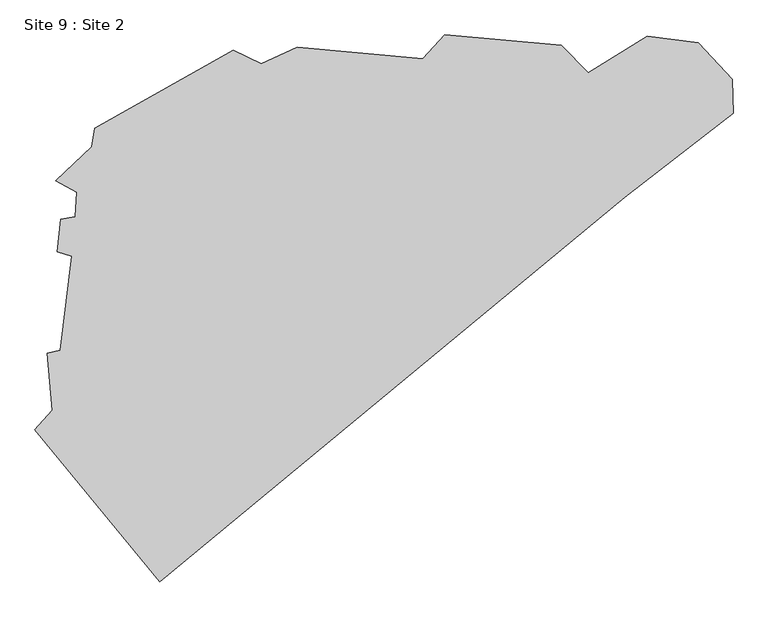
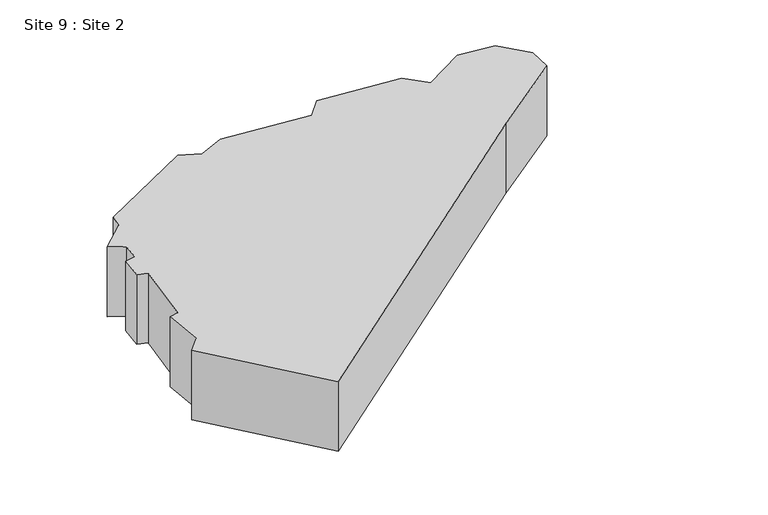
"""IFC4 building model written with IfcOpenShell, lengths in millimetres: geographic element geometry, Site 9 : Site 2."""

from ifc_helpers import new_model, si_unit, frame, origin, place, context, project, spatial, polyline, outline, extrude, source, transform, mapped, element, save


def site_9_site_2_4225363e(model_context):
    return source(origin(), model_context, "Body", "SweptSolid", [
        extrude(outline(polyline([(-52663.5762578, -39928.595116), (-61550.4941803, -29130.9188955), (-60310.8192275, -27726.3601163), (-60658.3068747, -23656.9457677), (-59741.0581441, -23467.0172822), (-58932.8015846, -16772.5268672), (-59944.2788523, -16453.0480066), (-59707.250861, -14119.4876127), (-58688.4150048, -13931.0308449), (-58561.8044455, -12205.5214874), (-60073.8708382, -11370.7058979), (-57498.8164451, -8969.4086212), (-57276.5056308, -7651.7194841), (-47441.5131213, -2104.0860833), (-45422.9695062, -3047.805243), (-42865.5757254, -1865.5534745), (-33936.0159808, -2706.1773326), (-32387.1560323, -1001.2724521), (-24065.6600225, -1731.4786944), (-22163.4249429, -3689.5973319), (-17959.9992411, -1108.6737776), (-14308.6691642, -1568.0052826), (-11907.3202968, -4143.0053853), (-11841.0507764, -6582.6105086), (-19548.5539567, -12567.4991584), (-52663.5762578, -39928.595116)])), frame((0.0, 0.0, 266395.2), z_axis=(0.0, 0.0, 1.0), x_axis=(1.0, 0.0, 0.0)), (0.0, 0.0, 1.0), 7620.0),
    ])


if __name__ == "__main__":
    model = new_model("IFC4")
    model_context = context("Model", 3, world=origin())
    ifc_project = project(units=[si_unit("LENGTHUNIT", "METRE", prefix="MILLI")], contexts=[model_context])
    site = spatial("IfcSite", under=ifc_project)
    building = spatial("IfcBuilding", under=site)
    placement = place(None, origin())
    site_9_site_2_shape = site_9_site_2_4225363e(model_context)
    element("IfcGeographicElement", 1, ObjectType="Site 9 : Site 2", at=placement, inside=building, context=model_context, shape_type="MappedRepresentation", body=[
        mapped(site_9_site_2_shape, transform((0.0, 0.0, 0.0), x_axis=(1.0, 0.0, 0.0), y_axis=(0.0, 1.0, 0.0), z_axis=(0.0, 0.0, 1.0))),
    ])
    save(model, "model.ifc")

# Revit data of these elements
# Element 1 (IfcGeographicElement, "Site 9 : Site 2")
#   Materials on its faces: "EXISTING BUILDING"
# Materials
#   "EXISTING BUILDING": class "Generic", colour RGB 120 120 120, transparency 0, Cost = 0
